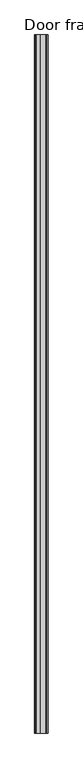
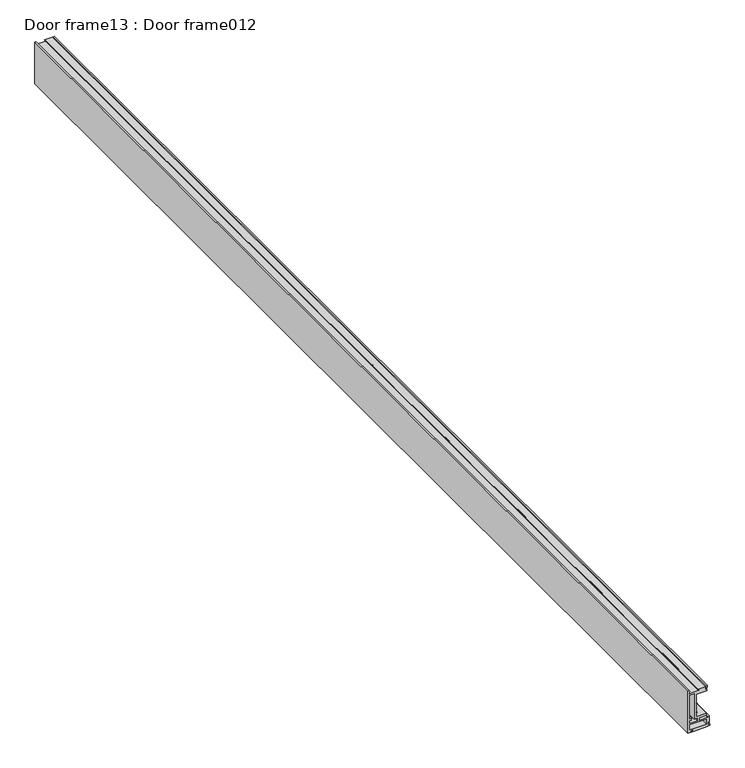
"""IFC4 building model written with IfcOpenShell, lengths in millimetres: proxy geometry, Door frame13 : Door frame012."""

from ifc_helpers import new_model, si_unit, frame, origin, place, context, project, spatial, polyline, outline, extrude, source, transform, mapped, element, save


def door_frame13_door_frame012_2ed3f318(model_context):
    return source(origin(), model_context, "Body", "SweptSolid", [
        extrude(outline(polyline([(36608.9977225, 15539.5084948), (36608.9977225, 15524.517453), (36613.8237225, 15524.517453), (36613.8237225, 15537.3384133), (36616.9987225, 15537.3384133), (36616.9987225, 15519.5076168), (36623.9157731, 15519.5076168), (36624.8727225, 15520.9106887), (36625.8290531, 15519.5076168), (36640.6803935, 15519.5076168), (36641.6367241, 15520.9106887), (36642.5936735, 15519.5076168), (36658.8030324, 15519.5076168), (36658.8030324, 15538.2476818), (36662.4618113, 15538.2476818), (36661.0188583, 15535.7484139), (36666.3421883, 15535.7484139), (36665.4690732, 15539.0049628), (36668.703989, 15539.288472), (36667.561659, 15536.9486127), (36667.7957063, 15535.7484139), (36667.7957063, 15522.1352688), (36666.5824658, 15522.1352688), (36666.5824658, 15523.6520602), (36664.6229889, 15523.6520602), (36664.6229889, 15506.8580308), (36666.7222221, 15506.8580308), (36668.7089205, 15508.0054504), (36669.4492947, 15507.5857589), (36669.4492947, 15504.8264133), (36591.6236909, 15504.8264133), (36591.6236909, 15510.4085802), (36592.8950628, 15510.4085802), (36592.8950628, 15509.5254133), (36594.1652793, 15509.5254133), (36594.1652793, 15514.0974128), (36592.8950628, 15514.0974128), (36592.8950628, 15513.2142459), (36591.6240434, 15513.2142459), (36591.6240434, 15540.1828722), (36593.5561506, 15540.1828722), (36593.5561506, 15541.3652071), (36592.4137824, 15543.7050664), (36595.6486981, 15543.4215572), (36594.775583, 15540.1650084), (36600.1211436, 15540.1650084), (36598.5843732, 15542.6834949), (36610.4200435, 15542.6834949), (36610.4200435, 15539.5084948), (36608.9977225, 15539.5084948)]), holes=[polyline([(36608.9977225, 15508.0061443), (36613.8237225, 15508.0061443), (36613.8237225, 15511.1764133), (36616.9987225, 15511.1764133), (36616.9987225, 15508.0014133), (36661.4479889, 15508.0014133), (36661.4479889, 15516.3326168), (36613.8237225, 15516.3326168), (36613.8237225, 15521.3411443), (36608.9977225, 15521.3411443), (36608.9977225, 15508.0061443)]), polyline([(36605.8183749, 15537.6432186), (36596.3988909, 15537.6432186), (36596.3988909, 15508.0014133), (36605.8183749, 15508.0014133), (36605.8183749, 15537.6432186)])]), frame((0.0, -1052.8906567, 0.0), z_axis=(0.0, 1.0, 0.0), x_axis=(0.0, 0.0, 1.0)), (0.0, 0.0, 1.0), 1999.85),
    ])


if __name__ == "__main__":
    model = new_model("IFC4")
    model_context = context("Model", 3, world=origin())
    ifc_project = project(units=[si_unit("LENGTHUNIT", "METRE", prefix="MILLI")], contexts=[model_context])
    site = spatial("IfcSite", under=ifc_project)
    building = spatial("IfcBuilding", under=site)
    placement = place(None, origin())
    door_frame13_door_frame012_shape = door_frame13_door_frame012_2ed3f318(model_context)
    element("IfcBuildingElementProxy", 1, Name="Door frame13 : Door frame012", ObjectType="Door frame13 : Door frame012", at=placement, inside=building, context=model_context, shape_type="MappedRepresentation", body=[
        mapped(door_frame13_door_frame012_shape, transform((0.0, 0.0, 0.0), x_axis=(1.0, 0.0, 0.0), y_axis=(0.0, 1.0, 0.0), z_axis=(0.0, 0.0, 1.0))),
    ])
    save(model, "model.ifc")

# Revit data of these elements
# Type "Door frame13 : Door frame012"
#   NameOverride = "Door frame012"
# Element 1 (IfcBuildingElementProxy, "Door frame13 : Door frame012")
#   Materials on its faces: "FLEETWOOD SERIES T-3200 SINGLE SWING DOOR FRAME"
# Materials
#   "FLEETWOOD SERIES T-3200 SINGLE SWING DOOR FRAME": class "Unassigned", colour RGB 128 128 128, transparency 0, Cost = 0
